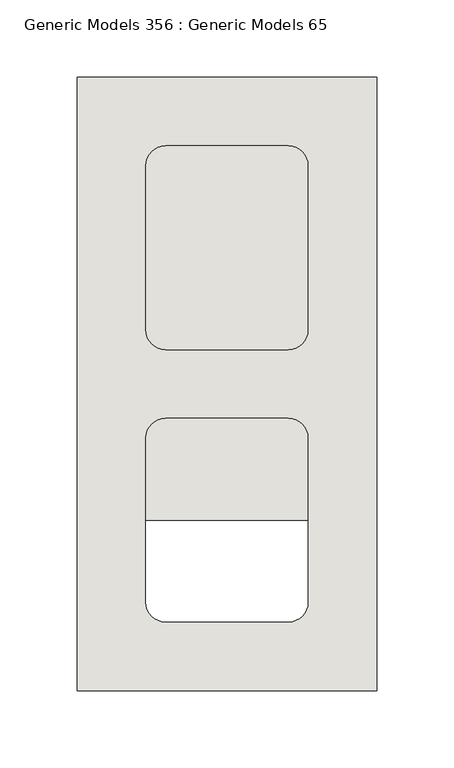
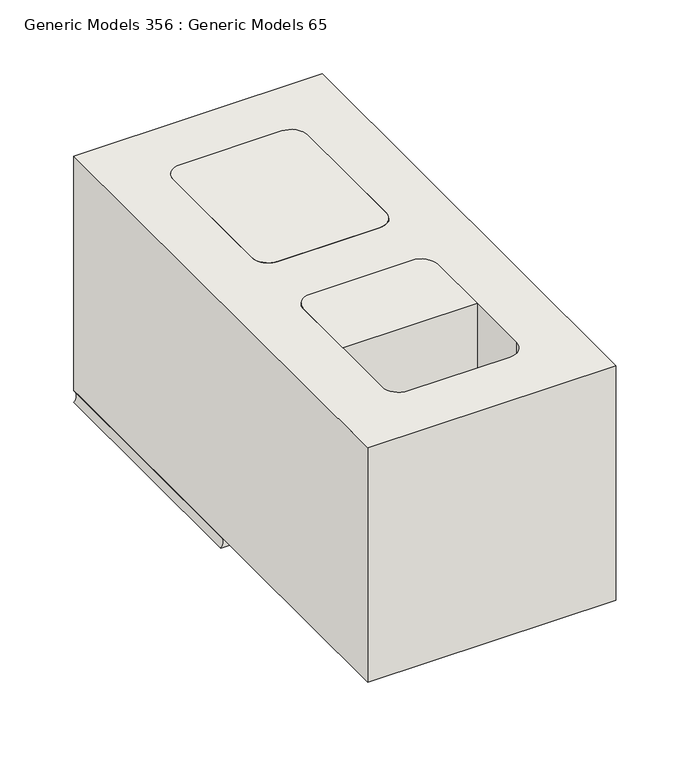
"""IFC4 building model written with IfcOpenShell, lengths in millimetres: wall geometry, Generic Models 356 : Generic Models 65."""

import ifcopenshell
import ifcopenshell.guid

model = None  # the IFC model being written
_history = None  # IfcOwnerHistory: only IFC2X3 demands one
_inside = {}  # id of a spatial element -> (the spatial element, [elements in it])
_under = {}  # id of a project, library or spatial element -> (it, [spatial elements below it])
_declared = {}  # id of a project -> (the project, [libraries it declares])
_typed = {}  # id of a type object -> (the type object, [elements of that type])
_made_of = {}  # id of a material, layer set ... -> (it, [elements and type objects made of it])


def new_model(schema):
    """Start an empty IFC model of exactly this schema.

    Asked for "IFC4X3", IfcOpenShell would pick the latest addendum, in which some entities
    have other attributes; the version numbers below select the first issue.
    IFC2X3 requires an IfcOwnerHistory on every rooted entity: one is made here for all.
    """
    global model, _history
    if schema == "IFC4X3":
        model = ifcopenshell.file(schema_version=(4, 3, 0, 0))
    else:
        model = ifcopenshell.file(schema=schema)
    _inside.clear()
    _under.clear()
    _declared.clear()
    _typed.clear()
    _made_of.clear()
    _history = None
    if model.schema == "IFC2X3":
        org = make("IfcOrganization", Name="unknown")
        user = make(
            "IfcPersonAndOrganization",
            ThePerson=make("IfcPerson", FamilyName="unknown"),
            TheOrganization=org,
        )
        app = make(
            "IfcApplication",
            ApplicationDeveloper=org,
            Version="unknown",
            ApplicationFullName="unknown",
            ApplicationIdentifier="unknown",
        )
        _history = make(
            "IfcOwnerHistory",
            OwningUser=user,
            OwningApplication=app,
            ChangeAction="ADDED",
            CreationDate=0,
        )
    return model


def make(cls, **values):
    """One entity of the class cls with the attributes given. An attribute that is None is left unset."""
    return model.create_entity(
        cls, **{name: value for name, value in values.items() if value is not None}
    )


def rooted(cls, **values):
    """An entity with a GlobalId (a new one), such as an element, a storey or a relation."""
    return make(cls, GlobalId=ifcopenshell.guid.new(), OwnerHistory=_history, **values)


def si_unit(unit_type, name, prefix=None):
    """IfcSIUnit, for example si_unit("LENGTHUNIT", "METRE", prefix="MILLI")."""
    return make("IfcSIUnit", UnitType=unit_type, Prefix=prefix, Name=name)


def assignment(units):
    """IfcUnitAssignment: the units of a project."""
    return None if units is None else make("IfcUnitAssignment", Units=units)


def point(xyz):
    """IfcCartesianPoint."""
    return None if xyz is None else make("IfcCartesianPoint", Coordinates=xyz)


def direction(xyz):
    """IfcDirection."""
    return None if xyz is None else make("IfcDirection", DirectionRatios=xyz)


def frame(location, z_axis=None, x_axis=None):
    """IfcAxis2Placement3D, a coordinate frame: its origin and axes. An axis left out is left unset."""
    return make(
        "IfcAxis2Placement3D",
        Location=point(location),
        Axis=direction(z_axis),
        RefDirection=direction(x_axis),
    )


def frame_2d(location, x_axis=None):
    """IfcAxis2Placement2D, a coordinate frame in the plane: its origin and x axis."""
    return make(
        "IfcAxis2Placement2D", Location=point(location), RefDirection=direction(x_axis)
    )


def origin():
    """The frame at (0, 0, 0) with its axes left unset."""
    return frame((0.0, 0.0, 0.0))


def place(relative_to, where):
    """IfcLocalPlacement: puts the frame where relative to a parent placement (None: the world)."""
    return make(
        "IfcLocalPlacement", PlacementRelTo=relative_to, RelativePlacement=where
    )


def context(
    kind, dimensions, precision=None, world=None, true_north=None, identifier=None
):
    """IfcGeometricRepresentationContext, for example the 3D "Model" context."""
    return make(
        "IfcGeometricRepresentationContext",
        ContextIdentifier=identifier,
        ContextType=kind,
        CoordinateSpaceDimension=dimensions,
        Precision=precision,
        WorldCoordinateSystem=world,
        TrueNorth=true_north,
    )


def project(units=None, contexts=None):
    """IfcProject with its units and contexts."""
    return rooted(
        "IfcProject",
        Name="project",
        RepresentationContexts=contexts,
        UnitsInContext=assignment(units),
    )


def spatial(cls, under=None, at=None, **own):
    """A site, building, storey or space (cls), placed at a placement, below another one or the project."""
    s = rooted(cls, ObjectPlacement=at, **own)
    if under is not None:
        _under.setdefault(under.id(), (under, []))[1].append(s)
    return s


def polyline(points):
    """IfcPolyline through the points."""
    return make("IfcPolyline", Points=[point(p) for p in points])


def circle_curve(where, radius):
    """IfcCircle in the frame where."""
    return make("IfcCircle", Position=where, Radius=radius)


def trimmed(basis, trim1, trim2, sense, master):
    """IfcTrimmedCurve: the piece of a basis curve between two trims."""
    return make(
        "IfcTrimmedCurve",
        BasisCurve=basis,
        Trim1=trim1,
        Trim2=trim2,
        SenseAgreement=sense,
        MasterRepresentation=master,
    )


def segment(curve, same_sense, transition):
    """IfcCompositeCurveSegment."""
    return make(
        "IfcCompositeCurveSegment",
        Transition=transition,
        SameSense=same_sense,
        ParentCurve=curve,
    )


def composite_curve(segments, self_intersect=None):
    """IfcCompositeCurve: segments joined end to end."""
    return make("IfcCompositeCurve", Segments=segments, SelfIntersect=self_intersect)


def outline(outer, holes=None, kind="AREA"):
    """IfcArbitraryClosedProfileDef: a profile drawn as a closed curve; with holes, ...WithVoids."""
    if holes is None:
        return make("IfcArbitraryClosedProfileDef", ProfileType=kind, OuterCurve=outer)
    return make(
        "IfcArbitraryProfileDefWithVoids",
        ProfileType=kind,
        OuterCurve=outer,
        InnerCurves=holes,
    )


def extrude(swept, where, along, depth):
    """IfcExtrudedAreaSolid: the profile swept, set in the frame where, extruded along a direction by depth."""
    return make(
        "IfcExtrudedAreaSolid",
        SweptArea=swept,
        Position=where,
        ExtrudedDirection=direction(along),
        Depth=depth,
    )


def shape(context_of_items, identifier, shape_type, items):
    """IfcShapeRepresentation: the items that make up one representation, for example the "Body"."""
    return make(
        "IfcShapeRepresentation",
        ContextOfItems=context_of_items,
        RepresentationIdentifier=identifier,
        RepresentationType=shape_type,
        Items=items,
    )


def source(mapping_origin, context_of_items, identifier, shape_type, items):
    """IfcRepresentationMap: a shape defined once, which mapped items show again and again."""
    return make(
        "IfcRepresentationMap",
        MappingOrigin=mapping_origin,
        MappedRepresentation=shape(context_of_items, identifier, shape_type, items),
    )


def transform(
    local_origin,
    x_axis=None,
    y_axis=None,
    z_axis=None,
    scale=None,
    scale2=None,
    scale3=None,
    uniform=True,
):
    """IfcCartesianTransformationOperator3D, or its non-uniform kind. x_axis, y_axis, z_axis: its Axis1, 2, 3."""
    if uniform:
        return make(
            "IfcCartesianTransformationOperator3D",
            Axis1=direction(x_axis),
            Axis2=direction(y_axis),
            LocalOrigin=point(local_origin),
            Scale=scale,
            Axis3=direction(z_axis),
        )
    return make(
        "IfcCartesianTransformationOperator3DnonUniform",
        Axis1=direction(x_axis),
        Axis2=direction(y_axis),
        LocalOrigin=point(local_origin),
        Scale=scale,
        Axis3=direction(z_axis),
        Scale2=scale2,
        Scale3=scale3,
    )


def mapped(mapping_source, mapping_target):
    """IfcMappedItem: shows the shape of a source again, moved by a transform."""
    return make(
        "IfcMappedItem", MappingSource=mapping_source, MappingTarget=mapping_target
    )


def made_of(thing, what):
    """Note that an element or type object is made of a material, layer set ...; save() writes the relation."""
    if what is not None:
        _made_of.setdefault(what.id(), (what, []))[1].append(thing)
    return thing


def element(
    cls,
    number,
    at=None,
    inside=None,
    cuts=None,
    type_object=None,
    material=None,
    context=None,
    identifier="Body",
    shape_type=None,
    held_by="IfcProductDefinitionShape",
    body=None,
    shapes=None,
    **own,
):
    """One element of the class cls, such as IfcWall. Its Tag is "e" and its number.

    at: its placement. inside: the storey or other place that contains it. cuts: it is an
    opening in that element (IfcRelVoidsElement). A single representation is given by context,
    identifier, shape_type and body (its items); several are given by shapes. held_by: the class
    of the entity that holds the representations. save() writes the other relations.
    """
    e = rooted(cls, Tag="e%d" % number, ObjectPlacement=at, **own)
    if body is not None:
        shapes = [shape(context, identifier, shape_type, body)]
    if shapes is not None:
        e.Representation = make(held_by, Representations=shapes)
    if inside is not None:
        _inside.setdefault(inside.id(), (inside, []))[1].append(e)
    if cuts is not None:
        rooted(
            "IfcRelVoidsElement", RelatingBuildingElement=cuts, RelatedOpeningElement=e
        )
    if type_object is not None:
        _typed.setdefault(type_object.id(), (type_object, []))[1].append(e)
    return made_of(e, material)


def aggregate(whole, parts):
    """IfcRelAggregates: a whole, such as a stair, and the parts it consists of."""
    return rooted("IfcRelAggregates", RelatingObject=whole, RelatedObjects=parts)


def save(model, path):
    """Write the relations noted so far, then the file.

    IfcRelAggregates (storeys below a building ...), IfcRelContainedInSpatialStructure (elements
    in a storey), IfcRelDefinesByType, IfcRelAssociatesMaterial and IfcRelDeclares: one each for
    every whole, place, type object, material and project.
    """
    for whole, parts in _under.values():
        aggregate(whole, parts)
    for where, things in _inside.values():
        rooted(
            "IfcRelContainedInSpatialStructure",
            RelatedElements=things,
            RelatingStructure=where,
        )
    for kind, things in _typed.values():
        rooted("IfcRelDefinesByType", RelatedObjects=things, RelatingType=kind)
    for what, things in _made_of.values():
        rooted("IfcRelAssociatesMaterial", RelatedObjects=things, RelatingMaterial=what)
    for by, libraries in _declared.values():
        rooted("IfcRelDeclares", RelatingContext=by, RelatedDefinitions=libraries)
    model.write(path)


def plane_surface(at):
    """IfcPlane: the flat surface through the origin of the frame at, square to its z axis."""
    return make("IfcPlane", Position=at)


def revolved_surface(curve, axis_point, axis_direction):
    """IfcSurfaceOfRevolution: the curve turned about the line through axis_point along axis_direction."""
    return make(
        "IfcSurfaceOfRevolution",
        SweptCurve=make("IfcArbitraryOpenProfileDef", ProfileType="CURVE", Curve=curve),
        AxisPosition=make("IfcAxis1Placement", Location=point(axis_point), Axis=direction(axis_direction)),
    )


def advanced_brep(points, edges, surfaces, faces):
    """IfcAdvancedBrep: a solid bounded by faces that lie on surfaces and meet in shared edges.

    An edge is (start, end): straight between two places in points (the first is 0);
    or (start, end, curve); or (start, end, curve, False) where it runs against its curve.
    A face is (place in surfaces, loops), or (place, loops, False) where it looks against
    its surface's normal. A loop lists edges by number (the first is 1), with a minus sign
    where the edge is run from its end to its start. The first loop is the outer one.
    """
    corners = [point(p) for p in points]
    vertices = [make("IfcVertexPoint", VertexGeometry=c) for c in corners]
    made = []
    for start, end, *more in edges:
        made.append(
            make(
                "IfcEdgeCurve",
                EdgeStart=vertices[start],
                EdgeEnd=vertices[end],
                EdgeGeometry=more[0] if more else make("IfcPolyline", Points=[corners[start], corners[end]]),
                SameSense=more[1] if len(more) > 1 else True,
            )
        )
    hull = []
    for where, loops, *sense in faces:
        bounds = []
        for j, loop in enumerate(loops):
            ring = [make("IfcOrientedEdge", EdgeElement=made[abs(k) - 1], Orientation=k > 0) for k in loop]
            bounds.append(
                make(
                    "IfcFaceOuterBound" if j == 0 else "IfcFaceBound",
                    Bound=make("IfcEdgeLoop", EdgeList=ring),
                    Orientation=True,
                )
            )
        hull.append(make("IfcAdvancedFace", Bounds=bounds, FaceSurface=surfaces[where], SameSense=sense[0] if sense else True))
    return make("IfcAdvancedBrep", Outer=make("IfcClosedShell", CfsFaces=hull))


def generic_models_356_generic_models_65_3847e57a(model_context):
    return source(origin(), model_context, "Body", "SolidModel", [
        advanced_brep(
        [(430198.2125, 503.2375, 415.925), (430004.5375, 503.2375, 415.925), (430004.5375, 503.2375, 406.4), (430198.2125, 503.2375, 406.4), (430198.2125, 701.675, 415.925), (430198.2125, 701.675, 406.4), (430004.5375, 701.675, 406.4), (430004.5375, 701.675, 415.925), (430153.7625, 538.1625, 415.925), (430141.0625, 525.4625, 415.925), (430061.6875, 525.4625, 415.925), (430048.9875, 538.1625, 415.925), (430048.9875, 644.525, 415.925), (430061.6875, 657.225, 415.925), (430141.0625, 657.225, 415.925), (430153.7625, 644.525, 415.925), (430141.0625, 525.4625, 406.4), (430153.7625, 538.1625, 406.4), (430061.6875, 525.4625, 406.4), (430048.9875, 538.1625, 406.4), (430048.9875, 644.525, 406.4), (430061.6875, 657.225, 406.4), (430141.0625, 657.225, 406.4), (430153.7625, 644.525, 406.4)],
        [
            (0, 1),
            (1, 2, circle_curve(frame((429999.6545028, 503.2375, 411.1625), z_axis=(0.0, 1.0, 0.0), x_axis=(1.0, 0.0, 0.0)), 6.8209287)),
            (2, 3),
            (3, 0, circle_curve(frame((430203.0954972, 503.2375, 411.1625), z_axis=(0.0, 1.0, 0.0), x_axis=(-1.0, 0.0, 0.0)), 6.8209287)),
            (4, 5, circle_curve(frame((430203.0954972, 701.675, 411.1625), z_axis=(0.0, -1.0, 0.0), x_axis=(-1.0, 0.0, 0.0)), 6.8209287)),
            (5, 6),
            (6, 7, circle_curve(frame((429999.6545028, 701.675, 411.1625), z_axis=(0.0, -1.0, 0.0), x_axis=(1.0, 0.0, 0.0)), 6.8209287)),
            (7, 4),
            (0, 4),
            (7, 1),
            (8, 9, circle_curve(frame((430141.0625, 538.1625, 415.925), z_axis=(0.0, 0.0, -1.0), x_axis=(-1.0, 0.0, 0.0)), 12.7)),
            (9, 10),
            (10, 11, circle_curve(frame((430061.6875, 538.1625, 415.925), z_axis=(0.0, 0.0, -1.0), x_axis=(-1.0, 0.0, 0.0)), 12.7)),
            (11, 12),
            (12, 13, circle_curve(frame((430061.6875, 644.525, 415.925), z_axis=(0.0, 0.0, -1.0), x_axis=(-1.0, 0.0, 0.0)), 12.7)),
            (13, 14),
            (14, 15, circle_curve(frame((430141.0625, 644.525, 415.925), z_axis=(0.0, 0.0, -1.0), x_axis=(-1.0, 0.0, 0.0)), 12.7)),
            (15, 8),
            (16, 9),
            (8, 17),
            (17, 16, circle_curve(frame((430141.0625, 538.1625, 406.4), z_axis=(0.0, 0.0, -1.0), x_axis=(-1.0, 0.0, 0.0)), 12.7)),
            (16, 18),
            (18, 10),
            (18, 19, circle_curve(frame((430061.6875, 538.1625, 406.4), z_axis=(0.0, 0.0, -1.0), x_axis=(-1.0, 0.0, 0.0)), 12.7)),
            (19, 11),
            (19, 20),
            (20, 12),
            (20, 21, circle_curve(frame((430061.6875, 644.525, 406.4), z_axis=(0.0, 0.0, -1.0), x_axis=(-1.0, 0.0, 0.0)), 12.7)),
            (21, 13),
            (21, 22),
            (22, 14),
            (22, 23, circle_curve(frame((430141.0625, 644.525, 406.4), z_axis=(0.0, 0.0, -1.0), x_axis=(-1.0, 0.0, 0.0)), 12.7)),
            (23, 15),
            (23, 17),
            (6, 2),
            (5, 3),
        ],
        [
            plane_surface(frame((430101.375, 503.2375, 416.321875), z_axis=(0.0, -1.0, 0.0), x_axis=(0.0, 0.0, 1.0))),
            plane_surface(frame((430101.375, 701.675, 416.321875), z_axis=(0.0, 1.0, 0.0), x_axis=(0.0, 0.0, 1.0))),
            plane_surface(frame((430198.2125, 503.2375, 415.925), z_axis=(0.0, 0.0, 1.0), x_axis=(0.0, 1.0, 0.0))),
            revolved_surface(polyline([(430128.3625, 538.1625, 415.925), (430128.3625, 538.1625, 406.4)]), (430141.0625, 538.1625, 600.075), (0.0, 0.0, 1.0)),
            plane_surface(frame((430061.6875, 525.4625, 600.075), z_axis=(0.0, 1.0, 0.0), x_axis=(0.0, 0.0, -1.0))),
            revolved_surface(polyline([(430048.9875, 538.1625, 415.925), (430048.9875, 538.1625, 406.4)]), (430061.6875, 538.1625, 600.075), (0.0, 0.0, 1.0)),
            plane_surface(frame((430048.9875, 644.525, 600.075), z_axis=(1.0, 0.0, 0.0), x_axis=(0.0, 0.0, -1.0))),
            revolved_surface(polyline([(430048.9875, 644.525, 415.925), (430048.9875, 644.525, 406.4)]), (430061.6875, 644.525, 600.075), (0.0, 0.0, 1.0)),
            plane_surface(frame((430141.0625, 657.225, 600.075), z_axis=(0.0, -1.0, 0.0), x_axis=(0.0, 0.0, -1.0))),
            revolved_surface(polyline([(430128.3625, 644.525, 415.925), (430128.3625, 644.525, 406.4)]), (430141.0625, 644.525, 600.075), (0.0, 0.0, 1.0)),
            plane_surface(frame((430153.7625, 538.1625, 600.075), z_axis=(-1.0, 0.0, 0.0), x_axis=(0.0, 0.0, -1.0))),
            revolved_surface(polyline([(430006.4754315, 701.675, 411.1625), (430006.4754315, 503.2375, 411.1625)]), (429999.6545028, 503.2375, 411.1625), (0.0, 1.0, 0.0)),
            plane_surface(frame((430004.5375, 503.2375, 406.4), z_axis=(0.0, 0.0, -1.0), x_axis=(0.0, 1.0, 0.0))),
            revolved_surface(polyline([(430196.2745685, 701.675, 411.1625), (430196.2745685, 503.2375, 411.1625)]), (430203.0954972, 503.2375, 411.1625), (0.0, 1.0, 0.0)),
        ],
        [
            (0, [[1, 2, 3, 4]]),
            (1, [[5, 6, 7, 8]]),
            (2, [[-1, 9, -8, 10], [11, 12, 13, 14, 15, 16, 17, 18]]),
            (3, [[19, -11, 20, 21]]),
            (4, [[-19, 22, 23, -12]]),
            (5, [[-23, 24, 25, -13]]),
            (6, [[-25, 26, 27, -14]]),
            (7, [[-27, 28, 29, -15]]),
            (8, [[-29, 30, 31, -16]]),
            (9, [[-31, 32, 33, -17]]),
            (10, [[-33, 34, -20, -18]]),
            (11, [[-2, -10, -7, 35]]),
            (12, [[-3, -35, -6, 36], [-21, -34, -32, -30, -28, -26, -24, -22]]),
            (13, [[-4, -36, -5, -9]]),
        ],
    ),
        extrude(outline(composite_curve([segment(trimmed(circle_curve(frame_2d((430141.0625, 538.1625)), 12.7), [point((430153.7625, 538.1625))], [point((430141.0625, 525.4625))], False, "CARTESIAN"), True, "CONTINUOUS"), segment(polyline([(430141.0625, 525.4625), (430061.6875, 525.4625)]), True, "CONTINUOUS"), segment(trimmed(circle_curve(frame_2d((430061.6875, 538.1625)), 12.7), [point((430061.6875, 525.4625))], [point((430048.9875, 538.1625))], False, "CARTESIAN"), True, "CONTINUOUS"), segment(polyline([(430048.9875, 538.1625), (430048.9875, 644.525)]), True, "CONTINUOUS"), segment(trimmed(circle_curve(frame_2d((430061.6875, 644.525)), 12.7), [point((430048.9875, 644.525))], [point((430061.6875, 657.225))], False, "CARTESIAN"), True, "CONTINUOUS"), segment(polyline([(430061.6875, 657.225), (430141.0625, 657.225)]), True, "CONTINUOUS"), segment(trimmed(circle_curve(frame_2d((430141.0625, 644.525)), 12.7), [point((430141.0625, 657.225))], [point((430153.7625, 644.525))], False, "CARTESIAN"), True, "CONTINUOUS"), segment(polyline([(430153.7625, 644.525), (430153.7625, 538.1625)]), True, "CONTINUOUS")], self_intersect=False)), frame((0.0, 0.0, 406.4), z_axis=(0.0, 0.0, 1.0), x_axis=(1.0, 0.0, 0.0)), (0.0, 0.0, 1.0), 203.2),
        extrude(outline(composite_curve([segment(trimmed(circle_curve(frame_2d((430061.6875, 468.3125)), 12.7), [point((430048.9875, 468.3125))], [point((430061.6875, 481.0125))], False, "CARTESIAN"), True, "CONTINUOUS"), segment(polyline([(430061.6875, 481.0125), (430141.0625, 481.0125)]), True, "CONTINUOUS"), segment(trimmed(circle_curve(frame_2d((430141.0625, 468.3125)), 12.7), [point((430141.0625, 481.0125))], [point((430153.7625, 468.3125))], False, "CARTESIAN"), True, "CONTINUOUS"), segment(polyline([(430153.7625, 468.3125), (430153.7625, 415.13125), (430048.9875, 415.13125), (430048.9875, 468.3125)]), True, "CONTINUOUS")], self_intersect=False)), frame((0.0, 0.0, 406.4), z_axis=(0.0, 0.0, 1.0), x_axis=(1.0, 0.0, 0.0)), (0.0, 0.0, 1.0), 203.2),
        extrude(outline(polyline([(430198.2125, 304.8), (430004.5375, 304.8), (430004.5375, 701.675), (430198.2125, 701.675), (430198.2125, 304.8)]), holes=[composite_curve([segment(polyline([(430153.7625, 538.1625), (430153.7625, 644.525)]), True, "CONTINUOUS"), segment(trimmed(circle_curve(frame_2d((430141.0625, 644.525)), 12.7), [point((430153.7625, 644.525))], [point((430141.0625, 657.225))], True, "CARTESIAN"), True, "CONTINUOUS"), segment(polyline([(430141.0625, 657.225), (430061.6875, 657.225)]), True, "CONTINUOUS"), segment(trimmed(circle_curve(frame_2d((430061.6875, 644.525)), 12.7), [point((430061.6875, 657.225))], [point((430048.9875, 644.525))], True, "CARTESIAN"), True, "CONTINUOUS"), segment(polyline([(430048.9875, 644.525), (430048.9875, 538.1625)]), True, "CONTINUOUS"), segment(trimmed(circle_curve(frame_2d((430061.6875, 538.1625)), 12.7), [point((430048.9875, 538.1625))], [point((430061.6875, 525.4625))], True, "CARTESIAN"), True, "CONTINUOUS"), segment(polyline([(430061.6875, 525.4625), (430141.0625, 525.4625)]), True, "CONTINUOUS"), segment(trimmed(circle_curve(frame_2d((430141.0625, 538.1625)), 12.7), [point((430141.0625, 525.4625))], [point((430153.7625, 538.1625))], True, "CARTESIAN"), True, "CONTINUOUS")], self_intersect=False), composite_curve([segment(polyline([(430048.9875, 468.3125), (430048.9875, 361.95)]), True, "CONTINUOUS"), segment(trimmed(circle_curve(frame_2d((430061.6875, 361.95)), 12.7), [point((430048.9875, 361.95))], [point((430061.6875, 349.25))], True, "CARTESIAN"), True, "CONTINUOUS"), segment(polyline([(430061.6875, 349.25), (430141.0625, 349.25)]), True, "CONTINUOUS"), segment(trimmed(circle_curve(frame_2d((430141.0625, 361.95)), 12.7), [point((430141.0625, 349.25))], [point((430153.7625, 361.95))], True, "CARTESIAN"), True, "CONTINUOUS"), segment(polyline([(430153.7625, 361.95), (430153.7625, 468.3125)]), True, "CONTINUOUS"), segment(trimmed(circle_curve(frame_2d((430141.0625, 468.3125)), 12.7), [point((430153.7625, 468.3125))], [point((430141.0625, 481.0125))], True, "CARTESIAN"), True, "CONTINUOUS"), segment(polyline([(430141.0625, 481.0125), (430061.6875, 481.0125)]), True, "CONTINUOUS"), segment(trimmed(circle_curve(frame_2d((430061.6875, 468.3125)), 12.7), [point((430061.6875, 481.0125))], [point((430048.9875, 468.3125))], True, "CARTESIAN"), True, "CONTINUOUS")], self_intersect=False)]), frame((0.0, 0.0, 415.925), z_axis=(0.0, 0.0, 1.0), x_axis=(1.0, 0.0, 0.0)), (0.0, 0.0, 1.0), 193.675),
    ])


if __name__ == "__main__":
    model = new_model("IFC4")
    model_context = context("Model", 3, world=origin())
    ifc_project = project(units=[si_unit("LENGTHUNIT", "METRE", prefix="MILLI")], contexts=[model_context])
    site = spatial("IfcSite", under=ifc_project)
    building = spatial("IfcBuilding", under=site)
    placement = place(None, origin())
    generic_models_356_generic_models_65_shape = generic_models_356_generic_models_65_3847e57a(model_context)
    element("IfcWall", 1, ObjectType="Generic Models 356 : Generic Models 65", at=placement, inside=building, context=model_context, shape_type="MappedRepresentation", body=[
        mapped(generic_models_356_generic_models_65_shape, transform((0.0, 0.0, 0.0), x_axis=(1.0, 0.0, 0.0), y_axis=(0.0, 1.0, 0.0), z_axis=(0.0, 0.0, 1.0))),
    ])
    save(model, "model.ifc")

# Revit data of these elements
# Element 1 (IfcWall, "Generic Models 356 : Generic Models 65")
#   Materials on its faces: "CMU (SEE 'WALL TAG' FOR SIZE)", "FILL CORE IF APPLICABLE - SEE STRUCTURAL DWGS FOR DETAILS", "MORTAR JOINT"
# Materials
#   "CMU (SEE 'WALL TAG' FOR SIZE)": class "Masonry", colour RGB 203 203 199, transparency 0, Description = "Concrete masonry units", Cost = 0
#   "FILL CORE IF APPLICABLE - SEE STRUCTURAL DWGS FOR DETAILS": class "Generic", colour RGB 170 170 170, transparency 0, Cost = 0
#   "MORTAR JOINT": class "Generic", colour RGB 120 120 120, transparency 0, Cost = 0
